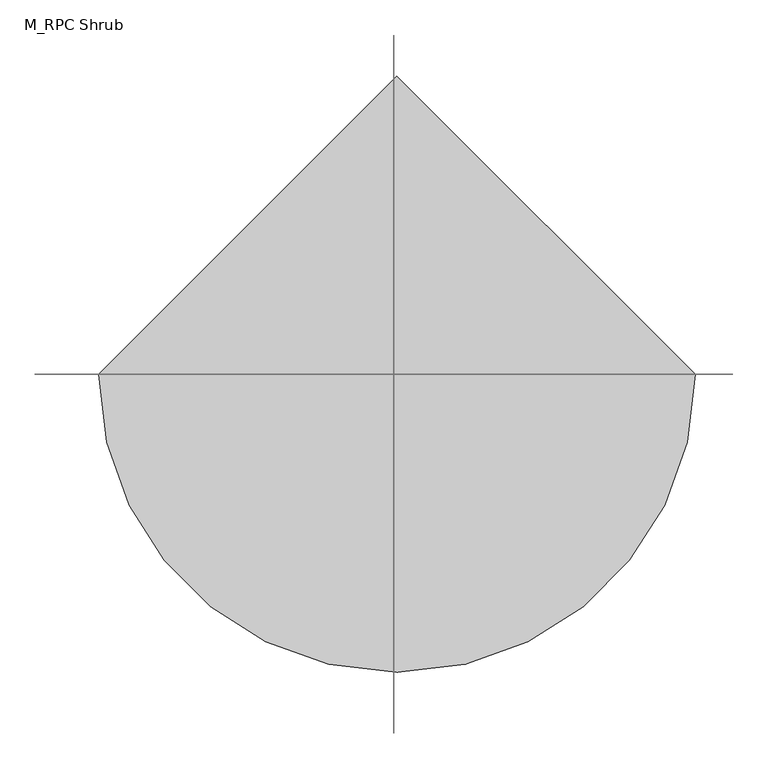
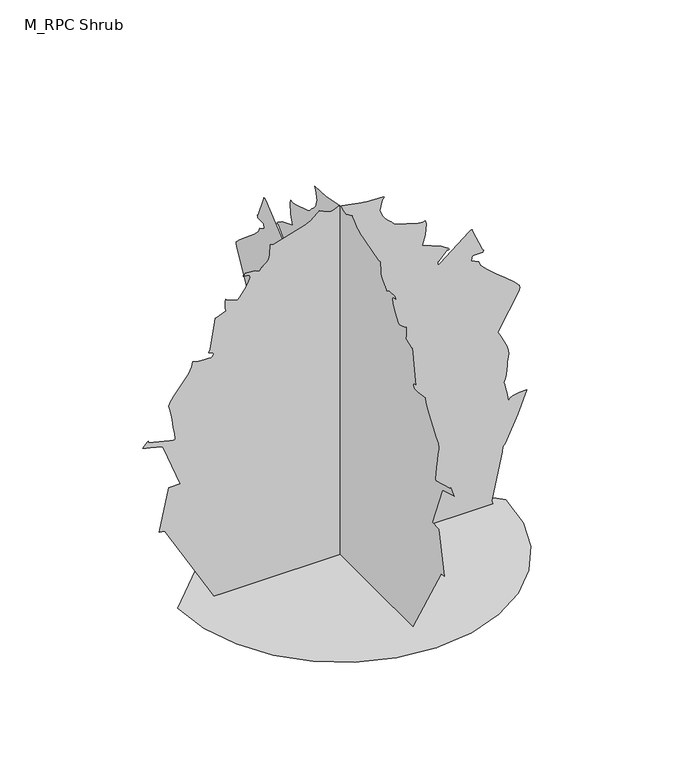
"""IFC4 building model written with IfcOpenShell, lengths in millimetres: geographic element geometry, M_RPC Shrub : Fraser Photina - 2.14 Meters."""

from ifc_helpers import new_model, si_unit, origin, place, context, project, spatial, triangles, source, transform, mapped, element, save


def m_rpc_shrub_1f038ad2(model_context):
    return source(origin(), model_context, "Body", "Tessellation", [
        triangles([(-946.0588234, 0.0, 1.51e-05), (-921.0487947, -216.7742865, 1.51e-05), (-849.8196396, -415.8466375, 1.51e-05), (-738.0731174, -591.5132043, 1.51e-05), (-591.5132043, -738.0731174, 1.51e-05), (-415.8466375, -849.8196396, 1.51e-05), (-216.7742865, -921.0487947, 1.51e-05), (4.14e-05, -946.0588234, 1.51e-05), (216.7742865, -921.0487947, 1.51e-05), (415.8466375, -849.8196396, 1.51e-05), (591.5132043, -738.0731174, 1.51e-05), (738.0731174, -591.5132043, 1.51e-05), (849.8196396, -415.8466375, 1.51e-05), (921.0487947, -216.7740322, 1.51e-05), (946.0588234, 8.27e-05, 1.51e-05), (-0.0001241, 946.0588234, 1.51e-05), (-1020.350219, 9.81e-05, 494.7823354), (-1053.4744326, 9.78e-05, 500.3030376), (-998.2647938, 8.26e-05, 754.2632629), (-932.0137505, 8.26e-05, 754.2632629), (-1031.3916235, 6.75e-05, 1008.2234882), (-1038.2268894, 6.7e-05, 1016.2689274), (-1135.8468756, 6.57e-05, 1042.5807661), (-1149.4308575, 6.54e-05, 1045.7831869), (-1147.3290236, 6.52e-05, 1046.8709839), (-1120.2579288, 6.58e-05, 1075.4859524), (-1116.2301224, 6.56e-05, 1077.7482416), (-1115.7231766, 6.51e-05, 1075.5496113), (-1116.8237635, 6.42e-05, 1068.4774412), (-1114.20481, 6.39e-05, 1068.953793), (-965.1405802, 6.62e-05, 1030.3088408), (-962.2362516, 6.56e-05, 1040.1681953), (-964.9367409, 6.38e-05, 1070.7932156), (-971.4077122, 6.12e-05, 1114.0620861), (-979.812359, 5.83e-05, 1161.8530643), (-988.3138023, 5.57e-05, 1206.0441896), (-995.0777063, 5.38e-05, 1238.5162628), (-998.2647938, 5.3e-05, 1251.1448524), (-989.4347368, 5.18e-05, 1271.5641003), (-968.5493111, 5.01e-05, 1300.6044788), (-940.6654753, 4.8e-05, 1335.3209644), (-910.8353193, 4.58e-05, 1372.7634464), (-884.1208889, 4.35e-05, 1409.9869011), (-865.5716578, 4.15e-05, 1444.0409271), (-860.2420412, 3.98e-05, 1471.9783207), (-844.7014927, 4.01e-05, 1468.2994755), (-825.2630716, 4.02e-05, 1465.3416618), (-804.2196613, 4.04e-05, 1463.0920898), (-783.8590582, 4.05e-05, 1461.5381149), (-766.4791597, 4.05e-05, 1460.6718887), (-754.3702332, 4.05e-05, 1460.4756798), (-749.8253071, 4.05e-05, 1460.9368435), (-744.2255762, 4.01e-05, 1466.8982529), (-740.6741941, 3.98e-05, 1472.9769516), (-739.5354555, 3.94e-05, 1478.8619122), (-741.1710388, 3.91e-05, 1484.2297531), (-745.9503256, 3.88e-05, 1488.7671215), (-754.2326689, 3.86e-05, 1492.1503452), (-766.3874502, 3.85e-05, 1494.0636005), (-759.2438456, 3.78e-05, 1514.1465317), (-739.3723841, 3.36e-05, 1637.0849579), (-734.2057663, 3.16e-05, 1673.3655922), (-730.2340611, 2.93e-05, 1694.5007847), (-727.742498, 2.67e-05, 1692.8142597), (-665.5472391, 2.54e-05, 1714.9302063), (-667.0121206, 2.54e-05, 1714.8996849), (-671.6691765, 2.58e-05, 1735.1532452), (-673.5952217, 2.51e-05, 1767.80881), (-672.2271366, 2.42e-05, 1778.7405556), (-670.2195557, 2.32e-05, 1785.096999), (-668.2528152, 2.22e-05, 1786.1440281), (-667.0121206, 2.14e-05, 1781.1481121), (-609.2599771, 2.26e-05, 1761.2536869), (-606.2817796, 2.27e-05, 1759.065303), (-602.3533493, 2.28e-05, 1757.1520477), (-589.1286115, 2.2e-05, 1770.4913498), (-552.0402503, 1.9e-05, 1822.3687065), (-536.802881, 1.73e-05, 1850.6219238), (-529.5217847, 1.59e-05, 1873.5607853), (-534.510034, 1.52e-05, 1886.0466511), (-568.2151351, 1.47e-05, 1894.2244949), (-568.6457047, 1.45e-05, 1894.9888378), (-561.4741221, 1.41e-05, 1900.7464806), (-556.5954228, 1.38e-05, 1908.1294601), (-500.0686406, 1.36e-05, 1903.3094055), (-473.7822364, 1.48e-05, 1891.5673897), (-469.5939383, 1.45e-05, 1897.1823086), (-466.4730895, 1.42e-05, 1901.7528145), (-463.8286652, 1.4e-05, 1905.5716221), (-461.0670241, 1.38e-05, 1908.9294113), (-457.5997212, 1.36e-05, 1912.1216583), (-452.8331154, 1.34e-05, 1915.438607), (-446.1761453, 1.32e-05, 1919.1709373), (-434.5385925, 1.27e-05, 1927.7131485), (-425.5352903, 1.19e-05, 1940.4027809), (-418.9649428, 1.1e-05, 1956.1981831), (-414.6288703, 9.9e-06, 1974.0595928), (-413.0518953, 6.6e-06, 2029.5902149), (-393.1345428, 6.7e-06, 2027.3788673), (-198.5671675, 3.3e-06, 2084.3361465), (-186.694709, 3e-06, 2090.3179035), (-180.7393857, 2.9e-06, 2091.5255333), (-140.8218822, 8e-07, 2126.2930332), (-134.061748, 3e-07, 2134.7435349), (-131.4858423, 0.0, 2140.0068764), (-83.0414429, 1.4e-06, 2116.5381054), (-69.3349485, 1.7e-06, 2112.6300591), (-55.12734, 1.7e-06, 2112.6198853), (-39.3830067, 1.4e-06, 2117.6769894), (-21.0679864, 7e-07, 2128.9655445), (133.9639251, 3.1e-06, 2098.2614594), (241.9868827, 5.2e-06, 2094.9240177), (245.4417227, 4.8e-06, 2090.8376392), (232.8928702, 3.6e-06, 2079.2765717), (219.5537498, 7.3e-06, 2017.3437241), (219.4266319, 7.6e-06, 2013.0383183), (221.8506845, 7.6e-06, 2013.0255283), (230.0657717, 9e-06, 1989.1338181), (238.8469399, 1e-05, 1971.9450417), (248.4193934, 1.08e-05, 1959.2196556), (259.0096264, 1.14e-05, 1948.7157909), (270.8433517, 1.21e-05, 1938.1940495), (284.1470637, 1.28e-05, 1925.4125622), (299.1423875, 1.38e-05, 1908.1294601), (309.8653522, 1.42e-05, 1902.2776371), (441.4528507, 1.66e-05, 1862.3792004), (468.2640776, 1.67e-05, 1859.5055386), (481.3334106, 1.65e-05, 1863.9612259), (486.7267224, 1.76e-05, 1844.8439335), (482.7192999, 2.17e-05, 1777.1381824), (464.7712675, 2.5e-05, 1720.4202782), (569.7080672, 2.52e-05, 1678.2775017), (614.4443991, 2.66e-05, 1648.7989231), (619.8988626, 2.75e-05, 1640.9241131), (617.0990335, 2.86e-05, 1638.7509899), (608.3122516, 2.96e-05, 1643.127903), (558.4806639, 3.28e-05, 1590.8786213), (553.1026128, 3.29e-05, 1587.9181915), (553.1026128, 3.42e-05, 1565.8353825), (568.4597059, 3.38e-05, 1573.3661728), (735.1458979, 2.78e-05, 1708.701226), (745.1707947, 2.83e-05, 1713.8831772), (750.3068184, 2.81e-05, 1715.2358562), (752.0468285, 2.75e-05, 1714.1099075), (751.8863005, 2.67e-05, 1711.8577194), (751.3258696, 2.6e-05, 1709.8273201), (751.8557791, 2.57e-05, 1709.3763302), (809.544191, 3.32e-05, 1575.167371), (818.1068224, 3.42e-05, 1565.8353825), (814.0535088, 3.44e-05, 1562.4062313), (814.2369278, 3.46e-05, 1559.4689106), (815.0317921, 3.47e-05, 1557.0995785), (812.817901, 3.48e-05, 1555.3697422), (751.8557791, 3.49e-05, 1554.7914345), (746.3350405, 3.66e-05, 1527.1878868), (790.5032747, 3.79e-05, 1505.1050777), (800.3625566, 3.93e-05, 1481.0122169), (836.6636839, 4.15e-05, 1443.5748219), (888.3525347, 4.42e-05, 1398.8333668), (944.3722984, 4.69e-05, 1352.8334129), (993.6740129, 4.94e-05, 1311.6179054), (1025.2008677, 5.12e-05, 1281.2271732), (1027.9013569, 5.2e-05, 1267.7069229), (1023.0888599, 5.31e-05, 1249.3564442), (900.9200089, 6.58e-05, 1035.8295794), (911.2633455, 6.69e-05, 1018.3732321), (924.2638601, 6.83e-05, 994.0026266), (937.9981236, 7e-05, 965.4641069), (950.5299168, 7.18e-05, 935.5116474), (959.935738, 7.35e-05, 906.8966789), (964.2870712, 7.5e-05, 882.370705), (961.6503136, 7.6e-05, 864.6825405), (956.8047518, 7.67e-05, 853.1417479), (954.603578, 7.78e-05, 835.8230375), (953.6430988, 7.9e-05, 814.2394712), (952.5119905, 8.05e-05, 789.9121771), (949.8064144, 8.2e-05, 764.3544348), (944.1200609, 8.35e-05, 739.0844656), (934.0467659, 8.49e-05, 715.6183107), (939.1088842, 8.55e-05, 705.9805996), (944.2398211, 8.66e-05, 687.5001143), (949.1720055, 8.8e-05, 663.9346195), (953.6430988, 8.95e-05, 639.0544521), (957.3906898, 9.08e-05, 616.6226091), (960.1472076, 9.18e-05, 600.4018696), (961.6503136, 9.22e-05, 594.1576286), (970.0116491, 9.13e-05, 608.4599896), (985.4247345, 9.07e-05, 618.4161043), (1025.7842623, 9.01e-05, 628.0639893), (1059.4715229, 9.01e-05, 628.6524708), (1066.5463091, 9.02e-05, 627.2844584), (1014.4218744, 9.8e-05, 495.877799), (942.6679693, 0.000107, 344.4239259), (928.5260273, 0.000108, 329.1559988), (927.2522678, 0.0001098, 297.9603012), (864.8150179, 0.0001263, 22.83981), (870.2872856, 0.0001276, 0.000103), (-735.9127115, 0.0001276, 0.000103), (-10.0261106, -1010.322706, 494.7823354), (-10.0261106, -1043.4469923, 500.3030376), (-10.0261106, -988.239897, 754.2632629), (-10.0261106, -921.9888536, 754.2632629), (-10.0260856, -1021.3641832, 1008.2234882), (-10.0260856, -1028.1994492, 1016.2689274), (-10.0260856, -1125.8194353, 1042.5807661), (-10.0260856, -1139.4033445, 1045.7831869), (-10.0260856, -1137.3041267, 1046.8709839), (-10.0260856, -1110.233032, 1075.4859524), (-10.0260856, -1106.2052256, 1077.7482416), (-10.0260856, -1105.6957363, 1075.5496113), (-10.0260856, -1106.7962505, 1068.4774412), (-10.0260856, -1104.177297, 1068.953793), (-10.0260856, -955.1156834, 1030.3088408), (-10.0260856, -952.2088114, 1040.1681953), (-10.0260856, -954.9093006, 1070.7932156), (-10.0260856, -961.3802719, 1114.0620861), (-10.0260856, -969.7849188, 1161.8530643), (-10.0260856, -978.2888329, 1206.0441896), (-10.0260856, -985.0502661, 1238.5162628), (-10.0260856, -988.239897, 1251.1448524), (-10.0260856, -979.4072966, 1271.5641003), (-10.0260856, -958.5217981, 1300.6044788), (-10.0260856, -930.638035, 1335.3209644), (-10.0260856, -900.8104225, 1372.7634464), (-10.0260856, -874.0959921, 1409.9869011), (-10.0260856, -855.5442175, 1444.0409271), (-10.0260856, -850.2170717, 1471.9783207), (-10.0260856, -834.6765959, 1468.2994755), (-10.0260856, -815.2381748, 1465.3416618), (-10.0260856, -794.1922211, 1463.0920898), (-10.0260856, -773.8341614, 1461.5381149), (-10.0260856, -756.4541903, 1460.6718887), (-10.0260856, -744.3453363, 1460.4756798), (-10.0260856, -739.8004103, 1460.9368435), (-10.0260856, -734.2006794, 1466.8982529), (-10.0260856, -730.6492973, 1472.9769516), (-10.0260856, -729.5079426, 1478.8619122), (-10.0260856, -731.1435259, 1484.2297531), (-10.0260856, -735.9228853, 1488.7671215), (-10.0260856, -744.2077721, 1492.1503452), (-10.0260856, -756.3624807, 1494.0636005), (-10.0260856, -749.2189487, 1514.1465317), (-10.0260856, -729.3474873, 1637.0849579), (-10.0260856, -724.1808695, 1673.3655922), (-10.0260856, -720.2091642, 1694.5007847), (-10.0260856, -717.7149851, 1692.8142597), (-10.0260856, -655.5223423, 1714.9302063), (-10.0260856, -656.9872238, 1714.8996849), (-10.0260856, -661.6442797, 1735.1532452), (-10.0260856, -663.5677088, 1767.80881), (-10.0260856, -662.1996237, 1778.7405556), (-10.0260856, -660.1921154, 1785.096999), (-10.0260856, -658.2279184, 1786.1440281), (-10.0260856, -656.9872238, 1781.1481121), (-10.0260856, -599.235044, 1761.2536869), (-10.0260856, -596.2568828, 1759.065303), (-10.0260856, -592.3258727, 1757.1520477), (-10.0260856, -579.1011349, 1770.4913498), (-10.0260856, -542.01281, 1822.3687065), (-10.0260856, -526.7779841, 1850.6219238), (-10.0260856, -519.4968515, 1873.5607853), (-10.0260856, -524.4851008, 1886.0466511), (-10.0260856, -558.1902383, 1894.2244949), (-10.0260595, -558.6207716, 1894.9888378), (-10.0260595, -551.449189, 1900.7464806), (-10.0260595, -546.5679462, 1908.1294601), (-10.0260856, -490.0437438, 1903.3094055), (-10.0260856, -463.7547961, 1891.5673897), (-10.0260856, -459.5690414, 1897.1823086), (-10.0260856, -456.4481927, 1901.7528145), (-10.0260856, -453.8011886, 1905.5716221), (-10.0260856, -451.0395839, 1908.9294113), (-10.0260856, -447.5722446, 1912.1216583), (-10.0260856, -442.8056388, 1915.438607), (-10.0260856, -436.1512485, 1919.1709373), (-10.0260856, -424.5136594, 1927.7131485), (-10.0260856, -415.5078137, 1940.4027809), (-10.0260856, -408.9374662, 1956.1981831), (-10.0260595, -404.60143, 1974.0595928), (-10.0260595, -403.0244551, 2029.5902149), (-10.0260595, -383.1071025, 2027.3788673), (-10.0260595, -188.5409808, 2084.3361465), (-10.0260595, -176.6687767, 2090.3179035), (-10.0260595, -170.7134534, 2091.5255333), (-10.0260595, -130.7959499, 2126.2930332), (-10.0260595, -124.0355613, 2134.7435349), (-10.0260595, -121.45991, 2140.0068764), (-10.0260856, -73.0152516, 2116.5381054), (-10.0260856, -59.3087618, 2112.6300591), (-10.0260856, -45.1014077, 2112.6198853), (-10.0260856, -29.3568177, 2117.6769894), (-10.0260856, -11.0419007, 2128.9655445), (-10.0260856, 143.9898575, 2098.2614594), (-10.0260856, 252.0130694, 2094.9240177), (-10.0260856, 255.4684181, 2090.8376392), (-10.0260856, 242.9188026, 2079.2765717), (-10.0260856, 229.5799366, 2017.3437241), (-10.0260856, 229.4525642, 2013.0383183), (-10.0260856, 231.8766169, 2013.0255283), (-10.0260856, 240.0919584, 1989.1338181), (-10.0260856, 248.8728723, 1971.9450417), (-10.0260856, 258.4465975, 1959.2196556), (-10.0260856, 269.0370848, 1948.7157909), (-10.0260856, 280.8682667, 1938.1940495), (-10.0260856, 294.1719787, 1925.4125622), (-10.0260856, 309.1698641, 1908.1294601), (-10.0260856, 319.8928288, 1902.2776371), (-10.0260856, 451.4803273, 1862.3792004), (-10.0260856, 478.2890107, 1859.5055386), (-10.0260856, 491.3583075, 1863.9612259), (-10.0260856, 496.7516556, 1844.8439335), (-10.0260856, 492.7467765, 1777.1381824), (-10.0260856, 474.7962007, 1720.4202782), (-10.0260856, 579.7355075, 1678.2775017), (-10.0260856, 624.4692959, 1648.7989231), (-10.0260856, 629.9237595, 1640.9241131), (-10.0260856, 627.1264738, 1638.7509899), (-10.0260856, 618.3397282, 1643.127903), (-10.0260856, 568.5055607, 1590.8786213), (-10.0260856, 563.1300894, 1587.9181915), (-10.0261106, 563.1300894, 1565.8353825), (-10.0261106, 578.4846391, 1573.3661728), (-10.0261106, 745.1707947, 1708.701226), (-10.0261106, 755.1982349, 1713.8831772), (-10.0261106, 760.3342587, 1715.2358562), (-10.0261106, 762.0717253, 1714.1099075), (-10.0261106, 761.9138134, 1711.8577194), (-10.0260856, 761.3507664, 1709.8273201), (-10.0260856, 761.8832193, 1709.3763302), (-10.0261106, 819.5717039, 1575.167371), (-10.0261106, 828.1342627, 1565.8353825), (-10.0261106, 824.0784056, 1562.4062313), (-10.0261106, 824.2618973, 1559.4689106), (-10.0261106, 825.059305, 1557.0995785), (-10.0261106, 822.8428705, 1555.3697422), (-10.0261106, 761.8832193, 1554.7914345), (-10.0261106, 756.3599373, 1527.1878868), (-10.0261106, 800.5281715, 1505.1050777), (-10.0261106, 810.3900696, 1481.0122169), (-10.0261106, 846.6911968, 1443.5748219), (-10.0261106, 898.3774315, 1398.8333668), (-10.0261106, 954.3997387, 1352.8334129), (-10.0261106, 1003.6989098, 1311.6179054), (-10.0261106, 1035.2283079, 1281.2271732), (-10.0261106, 1037.9262537, 1267.7069229), (-10.0261106, 1033.1138294, 1249.3564442), (-10.0261106, 910.9474491, 1035.8295794), (-10.0261106, 921.2882423, 1018.3732321), (-10.0261106, 934.2913731, 994.0026266), (-10.0261106, 948.0230204, 965.4641069), (-10.0261356, 960.557357, 935.5116474), (-10.0261356, 969.9632509, 906.8966789), (-10.0261356, 974.3120407, 882.370705), (-10.0261356, 971.6752104, 864.6825405), (-10.0261356, 966.832192, 853.1417479), (-10.0261356, 964.6310183, 835.8230375), (-10.0261356, 963.6680683, 814.2394712), (-10.0261356, 962.5394308, 789.9121771), (-10.0261356, 959.8338547, 764.3544348), (-10.0261356, 954.1475739, 739.0844656), (-10.0261356, 944.0716627, 715.6183107), (-10.0261356, 949.1338537, 705.9805996), (-10.0261356, 954.2647179, 687.5001143), (-10.0261356, 959.1969749, 663.9346195), (-10.0261356, 963.6706118, 639.0544521), (-10.0261356, 967.4155867, 616.6226091), (-10.0261356, 970.1721045, 600.4018696), (-10.0261356, 971.6752104, 594.1576286), (-10.0261356, 980.0365459, 608.4599896), (-10.0261356, 995.4522474, 618.4161043), (-10.0261356, 1035.8091591, 628.0639893), (-10.0261356, 1069.4990358, 628.6524708), (-10.0261356, 1076.5737494, 627.2844584), (-10.0261356, 1024.4493147, 495.877799), (-10.0261356, 952.6928661, 344.4239259), (-10.0261356, 938.5509968, 329.1559988), (-10.0261356, 937.2797081, 297.9603012), (-10.0261617, 874.8399147, 22.8397078), (-10.0261617, 880.3121824, 0.0), (-10.0261356, -725.8878147, 4.79e-05)], [[15, 16, 1], [14, 15, 1], [14, 1, 2], [13, 14, 2], [13, 2, 3], [13, 3, 4], [12, 13, 4], [11, 12, 4], [11, 4, 5], [11, 5, 6], [11, 6, 7], [11, 7, 8], [11, 8, 9], [11, 9, 10], [23, 24, 25], [62, 63, 64], [26, 27, 28], [70, 71, 72], [69, 70, 72], [196, 197, 198], [58, 59, 60], [97, 98, 99], [190, 191, 192], [127, 128, 129], [17, 18, 19], [44, 45, 46], [148, 149, 150], [25, 26, 28], [25, 28, 29], [23, 25, 29], [104, 105, 106], [23, 29, 30], [23, 30, 31], [22, 23, 31], [21, 22, 31], [20, 21, 31], [112, 113, 114], [111, 112, 114], [133, 134, 135], [133, 135, 136], [132, 133, 136], [81, 82, 83], [80, 81, 83], [17, 19, 20], [65, 66, 67], [80, 83, 84], [80, 84, 85], [189, 190, 192], [79, 80, 85], [116, 117, 118], [151, 152, 153], [195, 196, 198], [194, 195, 198], [194, 198, 17], [194, 17, 20], [194, 20, 31], [194, 31, 32], [188, 189, 192], [187, 188, 192], [186, 187, 192], [193, 194, 32], [192, 193, 32], [186, 192, 32], [185, 186, 32], [184, 185, 32], [183, 184, 32], [182, 183, 32], [181, 182, 32], [180, 181, 32], [179, 180, 32], [178, 179, 32], [177, 178, 32], [176, 177, 32], [175, 176, 32], [174, 175, 32], [173, 174, 32], [173, 32, 33], [173, 33, 34], [172, 173, 34], [171, 172, 34], [170, 171, 34], [169, 170, 34], [168, 169, 34], [167, 168, 34], [166, 167, 34], [165, 166, 34], [165, 34, 35], [165, 35, 36], [165, 36, 37], [165, 37, 38], [165, 38, 39], [165, 39, 40], [165, 40, 41], [165, 41, 42], [165, 42, 43], [165, 43, 44], [165, 44, 46], [165, 46, 47], [165, 47, 48], [165, 48, 49], [165, 49, 50], [165, 50, 51], [165, 51, 52], [165, 52, 53], [165, 53, 54], [165, 54, 55], [164, 165, 55], [163, 164, 55], [162, 163, 55], [161, 162, 55], [160, 161, 55], [159, 160, 55], [158, 159, 55], [157, 158, 55], [156, 157, 55], [155, 156, 55], [154, 155, 55], [154, 55, 56], [150, 151, 153], [148, 150, 153], [143, 144, 145], [142, 143, 145], [142, 145, 146], [141, 142, 146], [103, 104, 106], [132, 136, 137], [132, 137, 138], [68, 69, 72], [131, 132, 138], [148, 153, 154], [57, 58, 60], [67, 68, 72], [65, 67, 72], [65, 72, 73], [65, 73, 74], [65, 74, 75], [111, 114, 115], [78, 79, 85], [78, 85, 86], [111, 115, 116], [126, 127, 129], [154, 56, 57], [154, 57, 60], [154, 60, 61], [126, 129, 130], [126, 130, 131], [109, 110, 111], [141, 146, 147], [141, 147, 148], [141, 148, 154], [140, 141, 154], [62, 64, 65], [125, 126, 131], [111, 116, 118], [61, 62, 65], [131, 138, 139], [139, 140, 154], [139, 154, 61], [139, 61, 65], [139, 65, 75], [131, 139, 75], [131, 75, 76], [125, 131, 76], [124, 125, 76], [124, 76, 77], [123, 124, 77], [122, 123, 77], [121, 122, 77], [121, 77, 78], [121, 78, 86], [121, 86, 87], [120, 121, 87], [120, 87, 88], [120, 88, 89], [120, 89, 90], [120, 90, 91], [120, 91, 92], [120, 92, 93], [120, 93, 94], [120, 94, 95], [119, 120, 95], [119, 95, 96], [118, 119, 96], [111, 118, 96], [109, 111, 96], [108, 109, 96], [107, 108, 96], [106, 107, 96], [106, 96, 97], [102, 103, 106], [102, 106, 97], [101, 102, 97], [100, 101, 97], [100, 97, 99], [205, 206, 207], [244, 245, 246], [208, 209, 210], [252, 253, 254], [251, 252, 254], [378, 379, 380], [240, 241, 242], [279, 280, 281], [372, 373, 374], [309, 310, 311], [199, 200, 201], [226, 227, 228], [330, 331, 332], [207, 208, 210], [207, 210, 211], [205, 207, 211], [286, 287, 288], [205, 211, 212], [205, 212, 213], [204, 205, 213], [203, 204, 213], [202, 203, 213], [294, 295, 296], [293, 294, 296], [315, 316, 317], [315, 317, 318], [314, 315, 318], [263, 264, 265], [262, 263, 265], [199, 201, 202], [247, 248, 249], [262, 265, 266], [262, 266, 267], [371, 372, 374], [261, 262, 267], [298, 299, 300], [333, 334, 335], [377, 378, 380], [376, 377, 380], [376, 380, 199], [376, 199, 202], [376, 202, 213], [376, 213, 214], [370, 371, 374], [369, 370, 374], [368, 369, 374], [375, 376, 214], [374, 375, 214], [368, 374, 214], [367, 368, 214], [366, 367, 214], [365, 366, 214], [364, 365, 214], [363, 364, 214], [362, 363, 214], [361, 362, 214], [360, 361, 214], [359, 360, 214], [358, 359, 214], [357, 358, 214], [356, 357, 214], [355, 356, 214], [355, 214, 215], [355, 215, 216], [354, 355, 216], [353, 354, 216], [352, 353, 216], [351, 352, 216], [350, 351, 216], [349, 350, 216], [348, 349, 216], [347, 348, 216], [347, 216, 217], [347, 217, 218], [347, 218, 219], [347, 219, 220], [347, 220, 221], [347, 221, 222], [347, 222, 223], [347, 223, 224], [347, 224, 225], [347, 225, 226], [347, 226, 228], [347, 228, 229], [347, 229, 230], [347, 230, 231], [347, 231, 232], [347, 232, 233], [347, 233, 234], [347, 234, 235], [347, 235, 236], [347, 236, 237], [346, 347, 237], [345, 346, 237], [344, 345, 237], [343, 344, 237], [342, 343, 237], [341, 342, 237], [340, 341, 237], [339, 340, 237], [338, 339, 237], [337, 338, 237], [336, 337, 237], [336, 237, 238], [332, 333, 335], [330, 332, 335], [325, 326, 327], [324, 325, 327], [324, 327, 328], [323, 324, 328], [285, 286, 288], [314, 318, 319], [314, 319, 320], [250, 251, 254], [313, 314, 320], [330, 335, 336], [239, 240, 242], [249, 250, 254], [247, 249, 254], [247, 254, 255], [247, 255, 256], [247, 256, 257], [293, 296, 297], [260, 261, 267], [260, 267, 268], [293, 297, 298], [308, 309, 311], [336, 238, 239], [336, 239, 242], [336, 242, 243], [308, 311, 312], [308, 312, 313], [291, 292, 293], [323, 328, 329], [323, 329, 330], [323, 330, 336], [322, 323, 336], [244, 246, 247], [307, 308, 313], [293, 298, 300], [243, 244, 247], [313, 320, 321], [321, 322, 336], [321, 336, 243], [321, 243, 247], [321, 247, 257], [313, 321, 257], [313, 257, 258], [307, 313, 258], [306, 307, 258], [306, 258, 259], [305, 306, 259], [304, 305, 259], [303, 304, 259], [303, 259, 260], [303, 260, 268], [303, 268, 269], [302, 303, 269], [302, 269, 270], [302, 270, 271], [302, 271, 272], [302, 272, 273], [302, 273, 274], [302, 274, 275], [302, 275, 276], [302, 276, 277], [301, 302, 277], [301, 277, 278], [300, 301, 278], [293, 300, 278], [291, 293, 278], [290, 291, 278], [289, 290, 278], [288, 289, 278], [288, 278, 279], [284, 285, 288], [284, 288, 279], [283, 284, 279], [282, 283, 279], [282, 279, 281]], closed=False),
    ])


if __name__ == "__main__":
    model = new_model("IFC4")
    model_context = context("Model", 3, world=origin())
    ifc_project = project(units=[si_unit("LENGTHUNIT", "METRE", prefix="MILLI")], contexts=[model_context])
    site = spatial("IfcSite", under=ifc_project)
    building = spatial("IfcBuilding", under=site)
    placement = place(None, origin())
    m_rpc_shrub_shape = m_rpc_shrub_1f038ad2(model_context)
    element("IfcGeographicElement", 1, ObjectType="M_RPC Shrub : Fraser Photina - 2.14 Meters", at=placement, inside=building, context=model_context, shape_type="MappedRepresentation", body=[
        mapped(m_rpc_shrub_shape, transform((0.0, 0.0, 0.0), x_axis=(1.0, 0.0, 0.0), y_axis=(0.0, 1.0, 0.0), z_axis=(0.0, 0.0, 1.0))),
    ])
    save(model, "model.ifc")

# Revit data of these elements
# Type "M_RPC Shrub : Fraser Photina - 2.14 Meters"
#   Type Comments = "Fraser Photina"
#   built-in parameter 1005198 = "{2, 15},{39, RPC-16-G1TJ-U580-XE0H-6000-ST1L-LVER-AU},{1, 0},{1, 0},{2, 35},{1, 8},{5, Color},{1, 0},{1, 0},{3, 0.8},{3, 0.8},{3, 0.8},{1, 8},{7, BBoxMin},{1, 0},{1, 0},{1, 0},{1, 0},{1, 0},{1, 8},{7, BBoxMax},{1, 0},{1, 0},{1, 0},{1, 0},{1, 0},{2, 11},{9, RPCTypeId},{1, 0},{1, 0},{39, RPC-16-G1TJ-U580-XE0H-6000-ST1L-LVER-AU},{1, 6},{14, RPCPlantHeight},{1, 0},{1, 0},{5, 7.021},{2, 11},{7, keyword},{1, 0},{1, 0},{28, :Geometry:RPC:Fraser Photina},{2, 11},{8, category},{1, 0},{1, 0},{17, :Shrubs & Grasses},{2, 11},{12, LocalizedUID},{1, 0},{1, 0},{14, Fraser Photina},{2, 14},{6, Height},{1, 0},{1, 0},{5, 7.021},{1, 2},{16, Cast Reflections},{1, 0},{1, 0},{1, 0},{1, 2},{12, Cast Shadows},{1, 0},{1, 0},{1, 1},{1, 2},{9, Lock View},{1, 0},{1, 0},{1, 0},{1, 4},{5, ViewC},{1, 0},{1, 0},{1, 0},{2, 11},{20, AdvancedUIDefinition},{1, 0},{1, 0},{0, },{2, 11},{10, AssetLibID},{1, 0},{1, 0},{36, 4D3F6E72-3F99-4203-98E9-AF80B3C7A7A4},{2, 11},{10, BaseSchema},{1, 0},{1, 0},{9, RPCSchema},{2, 11},{12, ExchangeGUID},{1, 0},{1, 0},{0, },{1, 2},{6, Hidden},{1, 0},{1, 0},{1, 0},{1, 4},{11, RPCCategory},{1, 0},{1, 0},{1, 0},{2, 11},{8, RPCImage},{1, 0},{1, 0},{0, },{1, 4},{13, SchemaVersion},{1, 0},{1, 0},{1, 4},{2, 11},{12, UIDefinition},{1, 0},{1, 0},{0, },{2, 11},{6, UIName},{1, 0},{1, 0},{39, RPC-16-G1TJ-U580-XE0H-6000-ST1L-LVER-AU},{2, 11},{11, VersionGUID},{1, 0},{1, 0},{9, RPCSchema},{2, 11},{9, assettype},{1, 0},{1, 0},{11, RPCGeometry},{2, 11},{11, description},{1, 0},{1, 0},{0, },{2, 11},{9, localname},{1, 0},{1, 0},{3, RPC},{2, 11},{9, localtype},{1, 0},{1, 0},{3, RPC},{1, 4},{8, revision},{1, 0},{1, 0},{1, 1},{2, 11},{9, thumbnail},{1, 0},{1, 0},{0, },{1, 4},{7, version},{1, 0},{1, 0},{1, 1},{1, 2},{20, RPC_Cast Reflections},{1, 0},{1, 0},{1, 1},{1, 2},{16, RPC_Cast Shadows},{1, 0},{1, 0},{1, 1},{1, 2},{13, RPC_Lock View},{1, 0},{1, 0},{1, 0},{1, 4},{9, RPC_ViewC},{1, 0},{1, 0},{1, 0},{21, assetlibrary_base.fbx},{1, 5},"
#   built-in parameter 1005195 = "RPC-16-G1TJ-U580-XE0H-6000-ST1L-LVER-AU"
#   Height = 2.14 m
#   Description = (empty or 0)
#   Default Elevation = 0
